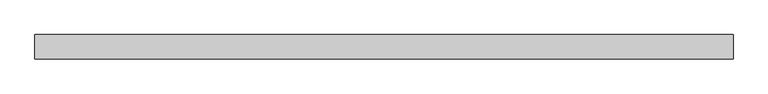
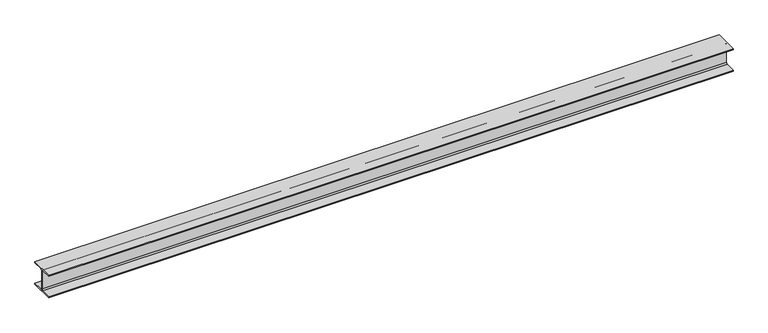
"""IFC4 building model written with IfcOpenShell, lengths in millimetres: beam geometry, 0912_Steel Framing_H-KSD3502 : H_SB_ASB_H-300x300x10x15."""

from ifc_helpers import new_model, si_unit, point, frame, frame_2d, origin, place, context, project, spatial, polyline, circle_curve, trimmed, segment, composite_curve, outline, extrude, source, transform, mapped, element, save


def beam_6708ffee(model_context):
    return source(origin(), model_context, "Body", "SweptSolid", [
        extrude(outline(composite_curve([segment(polyline([(150.0, -135.0), (150.0, -150.0), (-150.0, -150.0), (-150.0, -135.0), (-23.0, -135.0)]), True, "CONTINUOUS"), segment(trimmed(circle_curve(frame_2d((-23.0, -117.0)), 18.0), [point((-23.0, -135.0))], [point((-5.0, -117.0))], True, "CARTESIAN"), True, "CONTINUOUS"), segment(polyline([(-5.0, -117.0), (-5.0, 117.0)]), True, "CONTINUOUS"), segment(trimmed(circle_curve(frame_2d((-23.0, 117.0)), 18.0), [point((-5.0, 117.0))], [point((-23.0, 135.0))], True, "CARTESIAN"), True, "CONTINUOUS"), segment(polyline([(-23.0, 135.0), (-150.0, 135.0), (-150.0, 150.0), (150.0, 150.0), (150.0, 135.0), (23.0, 135.0)]), True, "CONTINUOUS"), segment(trimmed(circle_curve(frame_2d((23.0, 117.0)), 18.0), [point((23.0, 135.0))], [point((5.0, 117.0))], True, "CARTESIAN"), True, "CONTINUOUS"), segment(polyline([(5.0, 117.0), (5.0, -117.0)]), True, "CONTINUOUS"), segment(trimmed(circle_curve(frame_2d((23.0, -117.0)), 18.0), [point((5.0, -117.0))], [point((23.0, -135.0))], True, "CARTESIAN"), True, "CONTINUOUS"), segment(polyline([(23.0, -135.0), (150.0, -135.0)]), True, "CONTINUOUS")], self_intersect=False)), frame((-4272.9251782, 0.0, 0.0), z_axis=(1.0, 0.0, 0.0), x_axis=(0.0, 1.0, 0.0)), (0.0, 0.0, 1.0), 8596.9210734),
    ])


if __name__ == "__main__":
    model = new_model("IFC4")
    model_context = context("Model", 3, world=origin())
    ifc_project = project(units=[si_unit("LENGTHUNIT", "METRE", prefix="MILLI")], contexts=[model_context])
    site = spatial("IfcSite", under=ifc_project)
    building = spatial("IfcBuilding", under=site)
    placement = place(None, origin())
    beam_shape = beam_6708ffee(model_context)
    element("IfcBeam", 1, ObjectType="0912_Steel Framing_H-KSD3502 : H_SB_ASB_H-300x300x10x15", at=placement, inside=building, context=model_context, shape_type="MappedRepresentation", body=[
        mapped(beam_shape, transform((0.0, 0.0, 0.0), x_axis=(1.0, 0.0, 0.0), y_axis=(0.0, 1.0, 0.0), z_axis=(0.0, 0.0, 1.0))),
    ])
    save(model, "model.ifc")

# Revit data of these elements
# Type "0912_Steel Framing_H-KSD3502 : H_SB_ASB_H-300x300x10x15"
#   H_WM Code_1 = "S01AA001-00001 | Main Steel Structure Fabrication Work | Shelter/Building | Heavy Steel - Standard (Weight≥90KG/M) | Material: (   )"
#   H_WM Code_2 = "S03AA027-00001 | Main Steel Structure Erection Work | Shelter/Building | Heavy Steel (Weight≥90KG/M) | Material: (   )"
#   H_WM Code_3 = "S01AA010-00001 | Main Steel Structure Fabrication Work | Shelter/Building | Steel Painting/Coating | for Non-Fireproofed Steel Surface, Surface Preparation, Primer, Second & Final Coat | Material: (   )"
#   H_Q'ty Cal Type Tag = "SB-Q2"
#   Width = 30.0 cm
#   Web Thickness = 1.0 cm
#   Web Fillet = 1.8 cm
#   Warping Constant = 1370000.0 cm⁶
#   W = 0
#   Torsional Moment of Inertia = 77.00 cm⁴
#   Section Area = 119.8 cm²
#   Plastic Modulus weak axis = 684.0 cm³
#   Plastic Modulus strong axis = 1500.0 cm³
#   Perimeter = 1.75 m²/m
#   Nominal Weight = 94.00 kgf/m
#   Moment of Inertia weak axis = 6750.00 cm⁴
#   Moment of Inertia strong axis = 20400.00 cm⁴
#   Height = 30.0 cm
#   Flange Thickness = 1.5 cm
#   Elastic Modulus weak axis = 450.0 cm³
#   Elastic Modulus strong axis = 1360.0 cm³
#   Centroid Vertical = 15.0 cm
#   Centroid Horizontal = 15.0 cm
#   Ix = 204000000
#   Length [instance default] = 1.5240 m
#   Zx = 1500000
#   b = 0.3000 m
#   h = 0.3000 m
#   r = 0.0180 m
#   s = 0.0100 m
#   t = 0.0150 m
#   A = 0.01198 m²
#   Structural Material [instance default] = Steel, 45-345
#   Assembly Code = ""
# Element 1 (IfcBeam, "0912_Steel Framing_H-KSD3502 : H_SB_ASB_H-300x300x10x15")
#   Structural Material = none
# Materials
#   "Steel, 45-345": class "Metal", colour RGB 189 187 185, transparency 0, Description = "Steel 345 MPa", Cost = 0
